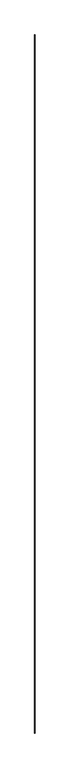
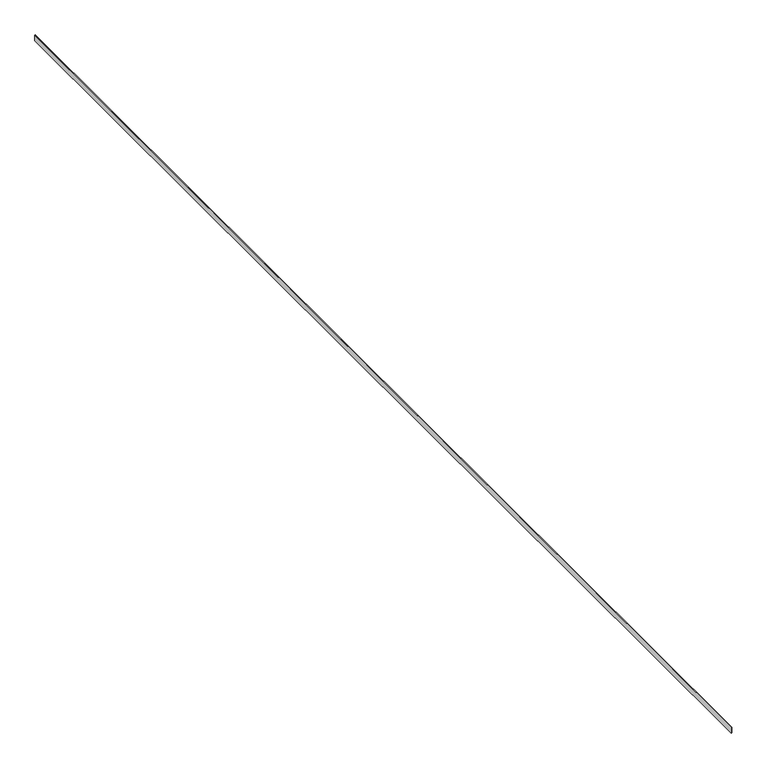
"""IFC4 building model written with IfcOpenShell, lengths in millimetres: proxy geometry, Generic Models 7:Generic Models 1:8:Generic Models 1:8 : Generic Models 7:Generic Models 1:337419:9 : Generic Models 7:Generic Models 1:8:Generic Models 1:8 : Generic Models 7:Generic Models 1:337419:315935."""

from ifc_helpers import new_model, si_unit, frame, origin, place, context, project, spatial, polyline, outline, extrude, source, transform, mapped, element, save


def generic_models_589d7458(model_context):
    return source(origin(), model_context, "Body", "SweptSolid", [
        extrude(outline(polyline([(3903.4402499, 560285.475475), (3903.4402499, 560270.4117208), (3720.3062499, 560270.4117208), (3720.3062499, 560286.2867208), (3902.6290041, 560286.2867208), (3903.4402499, 560285.475475)])), frame((0.0, -578670.4913841, 0.0), z_axis=(0.0, 1.0, 0.0), x_axis=(0.0, 0.0, 1.0)), (0.0, 0.0, 1.0), 35486.9749999),
    ])


if __name__ == "__main__":
    model = new_model("IFC4")
    model_context = context("Model", 3, world=origin())
    ifc_project = project(units=[si_unit("LENGTHUNIT", "METRE", prefix="MILLI")], contexts=[model_context])
    site = spatial("IfcSite", under=ifc_project)
    building = spatial("IfcBuilding", under=site)
    placement = place(None, origin())
    generic_models_shape = generic_models_589d7458(model_context)
    element("IfcBuildingElementProxy", 1, Name="Generic Models 7:Generic Models 1:8:Generic Models 1:8 : Generic Models 7:Generic Models 1:337419:9 : Generic Models 7:Generic Models 1:8:Generic Models 1:8 : Generic Models 7:Generic Models 1:337419:315935", ObjectType="Generic Models 7:Generic Models 1:8:Generic Models 1:8 : Generic Models 7:Generic Models 1:337419:9 : Generic Models 7:Generic Models 1:8:Generic Models 1:8 : Generic Models 7:Generic Models 1:337419:315935", at=placement, inside=building, context=model_context, shape_type="MappedRepresentation", body=[
        mapped(generic_models_shape, transform((0.0, 0.0, 0.0), x_axis=(1.0, 0.0, 0.0), y_axis=(0.0, 1.0, 0.0), z_axis=(0.0, 0.0, 1.0))),
    ])
    save(model, "model.ifc")

# Revit data of these elements
# Type "Generic Models 7:Generic Models 1:8:Generic Models 1:8 : Generic Models 7:Generic Models 1:337419:9 : Generic Models 7:Generic Models 1:8:Generic Models 1:8 : Generic Models 7:Generic Models 1:337419:315935"
#   NameOverride = "Generic Models 7:Generic Models 1:8:Generic Models 1:8 : Generic Models 7:Generic Models 1:337419:315935"
#   ObjectTypeOverride = "Generic Models 1:8 : Generic Models 7:Generic Models 1:337419"
#   Reference = "Generic Models 1"
#   Tag = "315935"
# Element 1 (IfcBuildingElementProxy, "Generic Models 7:Generic Models 1:8:Generic Models 1:8 : Generic Models 7:Generic Models 1:337419:9 : Generic Models 7:Generic Models 1:8:Generic Models 1:8 : Generic Models 7:Generic Models 1:337419:315935")
#   Materials on its faces: "ENGINEERED WOOD TRIM (LP SMARTSIDE)"
# Materials
#   "ENGINEERED WOOD TRIM (LP SMARTSIDE)": class "Wood", colour RGB 108 80 40, transparency 0, Description = "Pinus Echinata", Cost = 0
